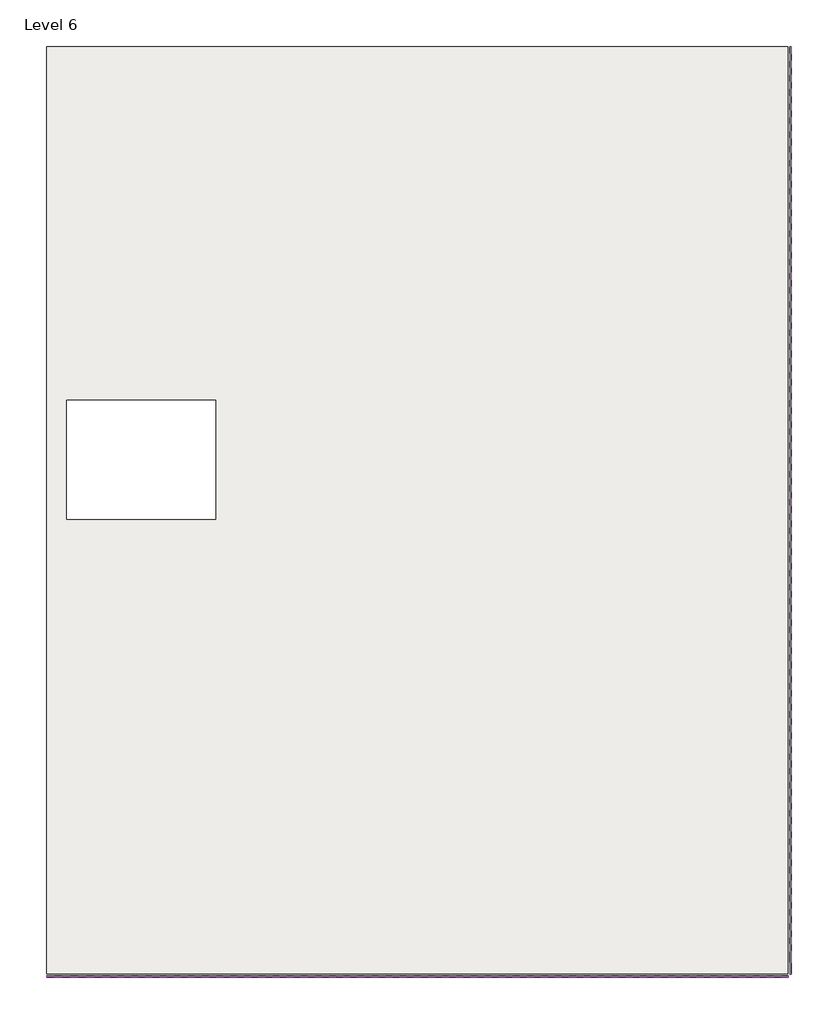
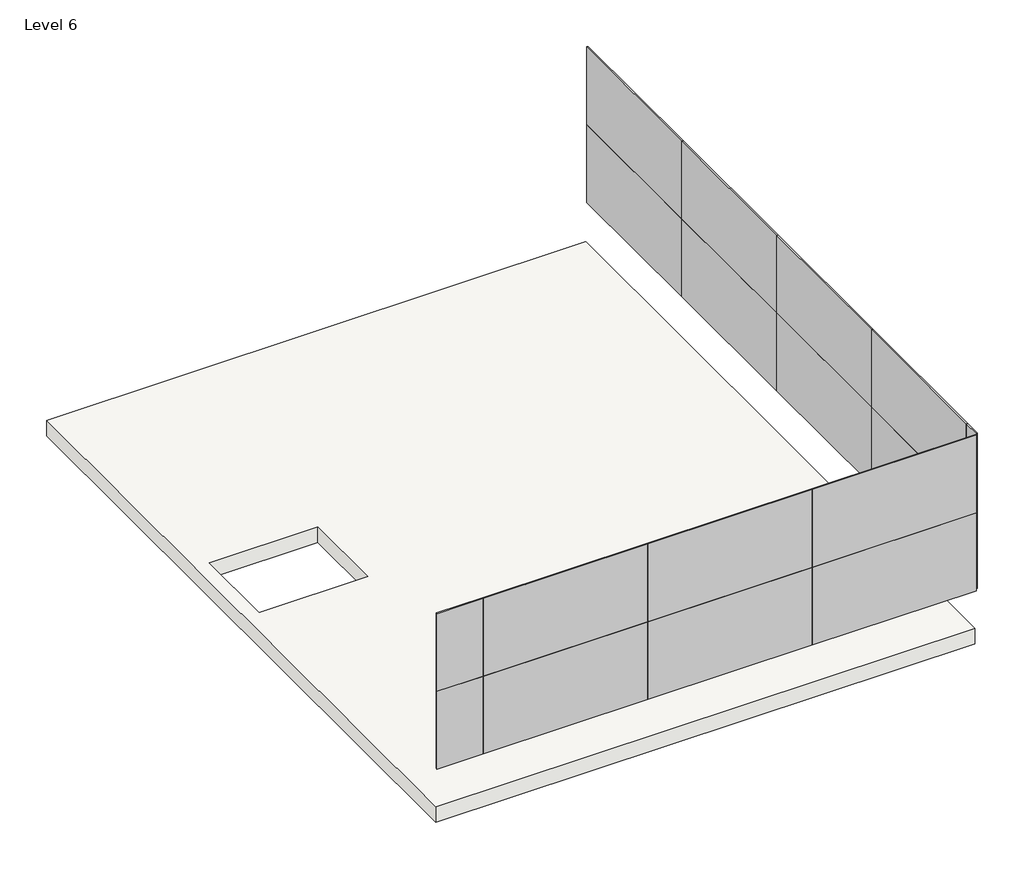
# One storey: 18 plates, 1 slab.
"""IFC4 building model written with IfcOpenShell, lengths in millimetres."""

import ifcopenshell
import ifcopenshell.guid

model = None  # the IFC model being written
_history = None  # IfcOwnerHistory: only IFC2X3 demands one
_inside = {}  # id of a spatial element -> (the spatial element, [elements in it])
_under = {}  # id of a project, library or spatial element -> (it, [spatial elements below it])
_declared = {}  # id of a project -> (the project, [libraries it declares])
_typed = {}  # id of a type object -> (the type object, [elements of that type])
_made_of = {}  # id of a material, layer set ... -> (it, [elements and type objects made of it])


def new_model(schema):
    """Start an empty IFC model of exactly this schema.

    Asked for "IFC4X3", IfcOpenShell would pick the latest addendum, in which some entities
    have other attributes; the version numbers below select the first issue.
    IFC2X3 requires an IfcOwnerHistory on every rooted entity: one is made here for all.
    """
    global model, _history
    if schema == "IFC4X3":
        model = ifcopenshell.file(schema_version=(4, 3, 0, 0))
    else:
        model = ifcopenshell.file(schema=schema)
    _inside.clear()
    _under.clear()
    _declared.clear()
    _typed.clear()
    _made_of.clear()
    _history = None
    if model.schema == "IFC2X3":
        org = make("IfcOrganization", Name="unknown")
        user = make(
            "IfcPersonAndOrganization",
            ThePerson=make("IfcPerson", FamilyName="unknown"),
            TheOrganization=org,
        )
        app = make(
            "IfcApplication",
            ApplicationDeveloper=org,
            Version="unknown",
            ApplicationFullName="unknown",
            ApplicationIdentifier="unknown",
        )
        _history = make(
            "IfcOwnerHistory",
            OwningUser=user,
            OwningApplication=app,
            ChangeAction="ADDED",
            CreationDate=0,
        )
    return model


def make(cls, **values):
    """One entity of the class cls with the attributes given. An attribute that is None is left unset."""
    return model.create_entity(
        cls, **{name: value for name, value in values.items() if value is not None}
    )


def rooted(cls, **values):
    """An entity with a GlobalId (a new one), such as an element, a storey or a relation."""
    return make(cls, GlobalId=ifcopenshell.guid.new(), OwnerHistory=_history, **values)


def si_unit(unit_type, name, prefix=None):
    """IfcSIUnit, for example si_unit("LENGTHUNIT", "METRE", prefix="MILLI")."""
    return make("IfcSIUnit", UnitType=unit_type, Prefix=prefix, Name=name)


def assignment(units):
    """IfcUnitAssignment: the units of a project."""
    return None if units is None else make("IfcUnitAssignment", Units=units)


def point(xyz):
    """IfcCartesianPoint."""
    return None if xyz is None else make("IfcCartesianPoint", Coordinates=xyz)


def direction(xyz):
    """IfcDirection."""
    return None if xyz is None else make("IfcDirection", DirectionRatios=xyz)


def frame(location, z_axis=None, x_axis=None):
    """IfcAxis2Placement3D, a coordinate frame: its origin and axes. An axis left out is left unset."""
    return make(
        "IfcAxis2Placement3D",
        Location=point(location),
        Axis=direction(z_axis),
        RefDirection=direction(x_axis),
    )


def origin():
    """The frame at (0, 0, 0) with its axes left unset."""
    return frame((0.0, 0.0, 0.0))


def origin_with_axes():
    """The frame at (0, 0, 0) with the z axis (0, 0, 1) and the x axis (1, 0, 0) written out."""
    return frame((0.0, 0.0, 0.0), z_axis=(0.0, 0.0, 1.0), x_axis=(1.0, 0.0, 0.0))


def place(relative_to, where):
    """IfcLocalPlacement: puts the frame where relative to a parent placement (None: the world)."""
    return make(
        "IfcLocalPlacement", PlacementRelTo=relative_to, RelativePlacement=where
    )


def context(
    kind, dimensions, precision=None, world=None, true_north=None, identifier=None
):
    """IfcGeometricRepresentationContext, for example the 3D "Model" context."""
    return make(
        "IfcGeometricRepresentationContext",
        ContextIdentifier=identifier,
        ContextType=kind,
        CoordinateSpaceDimension=dimensions,
        Precision=precision,
        WorldCoordinateSystem=world,
        TrueNorth=true_north,
    )


def project(units=None, contexts=None):
    """IfcProject with its units and contexts."""
    return rooted(
        "IfcProject",
        Name="project",
        RepresentationContexts=contexts,
        UnitsInContext=assignment(units),
    )


def spatial(cls, under=None, at=None, **own):
    """A site, building, storey or space (cls), placed at a placement, below another one or the project."""
    s = rooted(cls, ObjectPlacement=at, **own)
    if under is not None:
        _under.setdefault(under.id(), (under, []))[1].append(s)
    return s


def polyline(points):
    """IfcPolyline through the points."""
    return make("IfcPolyline", Points=[point(p) for p in points])


def outline(outer, holes=None, kind="AREA"):
    """IfcArbitraryClosedProfileDef: a profile drawn as a closed curve; with holes, ...WithVoids."""
    if holes is None:
        return make("IfcArbitraryClosedProfileDef", ProfileType=kind, OuterCurve=outer)
    return make(
        "IfcArbitraryProfileDefWithVoids",
        ProfileType=kind,
        OuterCurve=outer,
        InnerCurves=holes,
    )


def extrude(swept, where, along, depth):
    """IfcExtrudedAreaSolid: the profile swept, set in the frame where, extruded along a direction by depth."""
    return make(
        "IfcExtrudedAreaSolid",
        SweptArea=swept,
        Position=where,
        ExtrudedDirection=direction(along),
        Depth=depth,
    )


def shape(context_of_items, identifier, shape_type, items):
    """IfcShapeRepresentation: the items that make up one representation, for example the "Body"."""
    return make(
        "IfcShapeRepresentation",
        ContextOfItems=context_of_items,
        RepresentationIdentifier=identifier,
        RepresentationType=shape_type,
        Items=items,
    )


def source(mapping_origin, context_of_items, identifier, shape_type, items):
    """IfcRepresentationMap: a shape defined once, which mapped items show again and again."""
    return make(
        "IfcRepresentationMap",
        MappingOrigin=mapping_origin,
        MappedRepresentation=shape(context_of_items, identifier, shape_type, items),
    )


def transform(
    local_origin,
    x_axis=None,
    y_axis=None,
    z_axis=None,
    scale=None,
    scale2=None,
    scale3=None,
    uniform=True,
):
    """IfcCartesianTransformationOperator3D, or its non-uniform kind. x_axis, y_axis, z_axis: its Axis1, 2, 3."""
    if uniform:
        return make(
            "IfcCartesianTransformationOperator3D",
            Axis1=direction(x_axis),
            Axis2=direction(y_axis),
            LocalOrigin=point(local_origin),
            Scale=scale,
            Axis3=direction(z_axis),
        )
    return make(
        "IfcCartesianTransformationOperator3DnonUniform",
        Axis1=direction(x_axis),
        Axis2=direction(y_axis),
        LocalOrigin=point(local_origin),
        Scale=scale,
        Axis3=direction(z_axis),
        Scale2=scale2,
        Scale3=scale3,
    )


def mapped(mapping_source, mapping_target):
    """IfcMappedItem: shows the shape of a source again, moved by a transform."""
    return make(
        "IfcMappedItem", MappingSource=mapping_source, MappingTarget=mapping_target
    )


def made_of(thing, what):
    """Note that an element or type object is made of a material, layer set ...; save() writes the relation."""
    if what is not None:
        _made_of.setdefault(what.id(), (what, []))[1].append(thing)
    return thing


def element(
    cls,
    number,
    at=None,
    inside=None,
    cuts=None,
    type_object=None,
    material=None,
    context=None,
    identifier="Body",
    shape_type=None,
    held_by="IfcProductDefinitionShape",
    body=None,
    shapes=None,
    **own,
):
    """One element of the class cls, such as IfcWall. Its Tag is "e" and its number.

    at: its placement. inside: the storey or other place that contains it. cuts: it is an
    opening in that element (IfcRelVoidsElement). A single representation is given by context,
    identifier, shape_type and body (its items); several are given by shapes. held_by: the class
    of the entity that holds the representations. save() writes the other relations.
    """
    e = rooted(cls, Tag="e%d" % number, ObjectPlacement=at, **own)
    if body is not None:
        shapes = [shape(context, identifier, shape_type, body)]
    if shapes is not None:
        e.Representation = make(held_by, Representations=shapes)
    if inside is not None:
        _inside.setdefault(inside.id(), (inside, []))[1].append(e)
    if cuts is not None:
        rooted(
            "IfcRelVoidsElement", RelatingBuildingElement=cuts, RelatedOpeningElement=e
        )
    if type_object is not None:
        _typed.setdefault(type_object.id(), (type_object, []))[1].append(e)
    return made_of(e, material)


def aggregate(whole, parts):
    """IfcRelAggregates: a whole, such as a stair, and the parts it consists of."""
    return rooted("IfcRelAggregates", RelatingObject=whole, RelatedObjects=parts)


def save(model, path):
    """Write the relations noted so far, then the file.

    IfcRelAggregates (storeys below a building ...), IfcRelContainedInSpatialStructure (elements
    in a storey), IfcRelDefinesByType, IfcRelAssociatesMaterial and IfcRelDeclares: one each for
    every whole, place, type object, material and project.
    """
    for whole, parts in _under.values():
        aggregate(whole, parts)
    for where, things in _inside.values():
        rooted(
            "IfcRelContainedInSpatialStructure",
            RelatedElements=things,
            RelatingStructure=where,
        )
    for kind, things in _typed.values():
        rooted("IfcRelDefinesByType", RelatedObjects=things, RelatingType=kind)
    for what, things in _made_of.values():
        rooted("IfcRelAssociatesMaterial", RelatedObjects=things, RelatingMaterial=what)
    for by, libraries in _declared.values():
        rooted("IfcRelDeclares", RelatingContext=by, RelatedDefinitions=libraries)
    model.write(path)


def system_panel_glazed_1e57f9bb(model_context):
    return source(origin(), model_context, "Body", "SweptSolid", [
        extrude(outline(polyline([(1524.0000002, 19.05), (-1524.0000002, 19.05), (-1524.0000002, 44.45), (1524.0000002, 44.45), (1524.0000002, 19.05)])), origin_with_axes(), (0.0, 0.0, 1.0), 1524.0),
    ])


def system_panel_glazed_ccfd9adb(model_context):
    return source(origin(), model_context, "Body", "SweptSolid", [
        extrude(outline(polyline([(427.9999998, 19.05), (-427.9999998, 19.05), (-427.9999998, 44.45), (427.9999998, 44.45), (427.9999998, 19.05)])), origin_with_axes(), (0.0, 0.0, 1.0), 1524.0),
    ])


def system_panel_glazed_88f24eba(model_context):
    return source(origin(), model_context, "Body", "SweptSolid", [
        extrude(outline(polyline([(153.9999998, 19.05), (-153.9999998, 19.05), (-153.9999998, 44.45), (153.9999998, 44.45), (153.9999998, 19.05)])), origin_with_axes(), (0.0, 0.0, 1.0), 1524.0),
    ])


model = new_model("IFC4")

# Units and contexts
model_context = context("Model", 3, world=origin())
ifc_project = project(units=[si_unit("LENGTHUNIT", "METRE", prefix="MILLI")], contexts=[model_context])

# Site, building, storey
site = spatial("IfcSite", under=ifc_project)
building = spatial("IfcBuilding", under=site)
storey = spatial("IfcBuildingStorey", under=building, Name="Level 6", Elevation=16000.0)

# Plates
placement = place(None, origin())
system_panel_glazed_shape = system_panel_glazed_1e57f9bb(model_context)
element("IfcPlate", 1, ObjectType="System Panel : Glazed", at=placement, inside=storey, context=model_context, shape_type="MappedRepresentation", body=[
    mapped(system_panel_glazed_shape, transform((2137.6340362, 1399.6955828, 16764.0), x_axis=(-1.0, 0.0, 0.0), y_axis=(0.0, -1.0, 0.0), z_axis=(0.0, 0.0, 1.0))),
])
element("IfcPlate", 2, ObjectType="System Panel : Glazed", at=placement, inside=storey, context=model_context, shape_type="MappedRepresentation", body=[
    mapped(system_panel_glazed_shape, transform((-910.3659639, 1399.6955828, 16764.0), x_axis=(-1.0, 0.0, 0.0), y_axis=(0.0, -1.0, 0.0), z_axis=(0.0, 0.0, 1.0))),
])
element("IfcPlate", 3, ObjectType="System Panel : Glazed", at=placement, inside=storey, context=model_context, shape_type="MappedRepresentation", body=[
    mapped(system_panel_glazed_shape, transform((-3958.3659639, 1399.6955828, 16764.0), x_axis=(-1.0, 0.0, 0.0), y_axis=(0.0, -1.0, 0.0), z_axis=(0.0, 0.0, 1.0))),
])
element("IfcPlate", 4, ObjectType="System Panel : Glazed", at=placement, inside=storey, context=model_context, shape_type="MappedRepresentation", body=[
    mapped(system_panel_glazed_shape, transform((2137.6340362, 1399.6955828, 18288.0), x_axis=(-1.0, 0.0, 0.0), y_axis=(0.0, -1.0, 0.0), z_axis=(0.0, 0.0, 1.0))),
])
element("IfcPlate", 5, ObjectType="System Panel : Glazed", at=placement, inside=storey, context=model_context, shape_type="MappedRepresentation", body=[
    mapped(system_panel_glazed_shape, transform((-910.3659639, 1399.6955828, 18288.0), x_axis=(-1.0, 0.0, 0.0), y_axis=(0.0, -1.0, 0.0), z_axis=(0.0, 0.0, 1.0))),
])
element("IfcPlate", 6, ObjectType="System Panel : Glazed", at=placement, inside=storey, context=model_context, shape_type="MappedRepresentation", body=[
    mapped(system_panel_glazed_shape, transform((-3958.3659639, 1399.6955828, 18288.0), x_axis=(-1.0, 0.0, 0.0), y_axis=(0.0, -1.0, 0.0), z_axis=(0.0, 0.0, 1.0))),
])
element("IfcPlate", 7, ObjectType="System Panel : Glazed", at=placement, inside=storey, context=model_context, shape_type="MappedRepresentation", body=[
    mapped(system_panel_glazed_shape, transform((3661.6340364, 12375.6955827, 16764.0), x_axis=(0.0, -1.0, 0.0), y_axis=(1.0, 0.0, 0.0), z_axis=(0.0, 0.0, 1.0))),
])
element("IfcPlate", 8, ObjectType="System Panel : Glazed", at=placement, inside=storey, context=model_context, shape_type="MappedRepresentation", body=[
    mapped(system_panel_glazed_shape, transform((3661.6340364, 9327.6955825, 16764.0), x_axis=(0.0, -1.0, 0.0), y_axis=(1.0, 0.0, 0.0), z_axis=(0.0, 0.0, 1.0))),
])
element("IfcPlate", 9, ObjectType="System Panel : Glazed", at=placement, inside=storey, context=model_context, shape_type="MappedRepresentation", body=[
    mapped(system_panel_glazed_shape, transform((3661.6340364, 6279.6955825, 16764.0), x_axis=(0.0, -1.0, 0.0), y_axis=(1.0, 0.0, 0.0), z_axis=(0.0, 0.0, 1.0))),
])
element("IfcPlate", 10, ObjectType="System Panel : Glazed", at=placement, inside=storey, context=model_context, shape_type="MappedRepresentation", body=[
    mapped(system_panel_glazed_shape, transform((3661.6340364, 3231.6955825, 16764.0), x_axis=(0.0, -1.0, 0.0), y_axis=(1.0, 0.0, 0.0), z_axis=(0.0, 0.0, 1.0))),
])
element("IfcPlate", 11, ObjectType="System Panel : Glazed", at=placement, inside=storey, context=model_context, shape_type="MappedRepresentation", body=[
    mapped(system_panel_glazed_shape, transform((3661.6340364, 12375.6955827, 18288.0), x_axis=(0.0, -1.0, 0.0), y_axis=(1.0, 0.0, 0.0), z_axis=(0.0, 0.0, 1.0))),
])
element("IfcPlate", 12, ObjectType="System Panel : Glazed", at=placement, inside=storey, context=model_context, shape_type="MappedRepresentation", body=[
    mapped(system_panel_glazed_shape, transform((3661.6340364, 9327.6955825, 18288.0), x_axis=(0.0, -1.0, 0.0), y_axis=(1.0, 0.0, 0.0), z_axis=(0.0, 0.0, 1.0))),
])
element("IfcPlate", 13, ObjectType="System Panel : Glazed", at=placement, inside=storey, context=model_context, shape_type="MappedRepresentation", body=[
    mapped(system_panel_glazed_shape, transform((3661.6340364, 6279.6955825, 18288.0), x_axis=(0.0, -1.0, 0.0), y_axis=(1.0, 0.0, 0.0), z_axis=(0.0, 0.0, 1.0))),
])
element("IfcPlate", 14, ObjectType="System Panel : Glazed", at=placement, inside=storey, context=model_context, shape_type="MappedRepresentation", body=[
    mapped(system_panel_glazed_shape, transform((3661.6340364, 3231.6955825, 18288.0), x_axis=(0.0, -1.0, 0.0), y_axis=(1.0, 0.0, 0.0), z_axis=(0.0, 0.0, 1.0))),
])
system_panel_glazed_2_shape = system_panel_glazed_ccfd9adb(model_context)
element("IfcPlate", 15, ObjectType="System Panel : Glazed", at=placement, inside=storey, context=model_context, shape_type="MappedRepresentation", body=[
    mapped(system_panel_glazed_2_shape, transform((-5910.3659638, 1399.6955828, 16764.0), x_axis=(-1.0, 0.0, 0.0), y_axis=(0.0, -1.0, 0.0), z_axis=(0.0, 0.0, 1.0))),
])
element("IfcPlate", 16, ObjectType="System Panel : Glazed", at=placement, inside=storey, context=model_context, shape_type="MappedRepresentation", body=[
    mapped(system_panel_glazed_2_shape, transform((-5910.3659638, 1399.6955828, 18288.0), x_axis=(-1.0, 0.0, 0.0), y_axis=(0.0, -1.0, 0.0), z_axis=(0.0, 0.0, 1.0))),
])
system_panel_glazed_3_shape = system_panel_glazed_88f24eba(model_context)
element("IfcPlate", 17, ObjectType="System Panel : Glazed", at=placement, inside=storey, context=model_context, shape_type="MappedRepresentation", body=[
    mapped(system_panel_glazed_3_shape, transform((3661.6340364, 1553.6955827, 16764.0), x_axis=(0.0, -1.0, 0.0), y_axis=(1.0, 0.0, 0.0), z_axis=(0.0, 0.0, 1.0))),
])
element("IfcPlate", 18, ObjectType="System Panel : Glazed", at=placement, inside=storey, context=model_context, shape_type="MappedRepresentation", body=[
    mapped(system_panel_glazed_3_shape, transform((3661.6340364, 1553.6955827, 18288.0), x_axis=(0.0, -1.0, 0.0), y_axis=(1.0, 0.0, 0.0), z_axis=(0.0, 0.0, 1.0))),
])

# Slab
element("IfcSlab", 19, ObjectType="Generic - 12\"", at=placement, inside=storey, context=model_context, shape_type="SweptSolid", body=[
    extrude(outline(polyline([(-6335.3659636, 1402.6955828), (-6335.3659636, 13896.6955828), (3658.6340364, 13896.6955828), (3658.6340364, 1402.6955828), (-6335.3659636, 1402.6955828)]), holes=[polyline([(-4059.8993101, 7527.9023719), (-4059.8993101, 9133.9023719), (-6065.8993101, 9133.9023719), (-6065.8993101, 7527.9023719), (-4059.8993101, 7527.9023719)])]), frame((0.0, 0.0, 15695.2), z_axis=(0.0, 0.0, 1.0), x_axis=(1.0, 0.0, 0.0)), (0.0, 0.0, 1.0), 304.8),
])

save(model, "model.ifc")

# Revit data of these elements
# Type "System Panel : Glazed"
#   Construction Type Id = "GSP4R"
#   Analytic Construction = "1/8 in Pilkington single glazing"
#   Visual Light Transmittance = 0.9
#   Solar Heat Gain Coefficient = 0.86
#   Heat Transfer Coefficient (U) = 6.7069 W/(m²·K)
# Type "Generic - 12\""
#   Assembly Code = "B1010"
#   Function = 0
#   Layers, outside or top first: 0.3048 m no material (function 1)
# Elements 1, 2, 3, 4, 5, 6, 7, 8, 9, 10, 11, 12, 13, 14, 15, 16, 17, 18 (IfcPlate, "System Panel : Glazed")
#   Phase Created = New Construction
#   Materials on its faces: "Glass"
# Element 19 (IfcSlab, "Generic - 12\"")
#   built-in parameter 1001955 = -1.5708 (stored number, unit not read)
#   Height Offset From Level = 0.00 m
#   Phase Created = New Construction
#   Materials on its faces: "Default Floor"
# Materials
#   "Glass": class "Glass", colour RGB 0 128 192, transparency 0.75, Description = "Soda Lime Glass", Cost = 0
#   "Default Floor": class "Miscellaneous", colour RGB 128 128 128, transparency 0, Cost = 0
